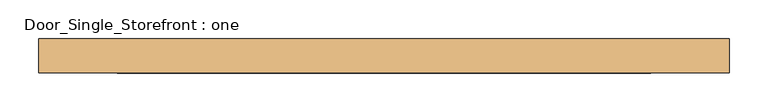
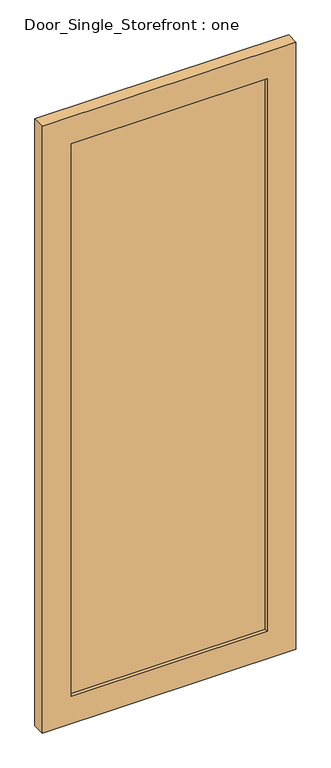
"""IFC4 building model written with IfcOpenShell, lengths in millimetres: door geometry, Door_Single_Storefront : one."""

from ifc_helpers import new_model, si_unit, frame, origin, place, context, project, spatial, polyline, outline, extrude, source, transform, mapped, element, save


def door_single_storefront_one_33456f2b(model_context):
    return source(origin(), model_context, "Body", "SweptSolid", [
        extrude(outline(polyline([(345.28125, -6.35), (-345.28125, -6.35), (-345.28125, 12.7), (345.28125, 12.7), (345.28125, -6.35)])), frame((0.0, 0.0, 101.6), z_axis=(0.0, 0.0, 1.0), x_axis=(1.0, 0.0, 0.0)), (0.0, 0.0, 1.0), 2057.4),
        extrude(outline(polyline([(2260.6, -446.88125), (0.0, -446.88125), (0.0, 446.88125), (2260.6, 446.88125), (2260.6, -446.88125)]), holes=[polyline([(101.6, 345.28125), (101.6, -345.28125), (2159.0, -345.28125), (2159.0, 345.28125), (101.6, 345.28125)])]), frame((0.0, -19.05, 0.0), z_axis=(0.0, 1.0, 0.0), x_axis=(0.0, 0.0, 1.0)), (0.0, 0.0, 1.0), 44.45),
    ])


if __name__ == "__main__":
    model = new_model("IFC4")
    model_context = context("Model", 3, world=origin())
    ifc_project = project(units=[si_unit("LENGTHUNIT", "METRE", prefix="MILLI")], contexts=[model_context])
    site = spatial("IfcSite", under=ifc_project)
    building = spatial("IfcBuilding", under=site)
    placement = place(None, origin())
    door_single_storefront_one_shape = door_single_storefront_one_33456f2b(model_context)
    element("IfcDoor", 1, ObjectType="Door_Single_Storefront : one", at=placement, inside=building, context=model_context, shape_type="MappedRepresentation", body=[
        mapped(door_single_storefront_one_shape, transform((0.0, 0.0, 0.0), x_axis=(1.0, 0.0, 0.0), y_axis=(0.0, 1.0, 0.0), z_axis=(0.0, 0.0, 1.0))),
    ])
    save(model, "model.ifc")

# Revit data of these elements
# Type "Door_Single_Storefront : one"
#   Type Mark = "27"
#   Analytic Construction = "<None>"
#   Stile_Width = 0' - 4"
#   Door_Thickness = 0' - 1 3/4"
#   Door_Offset = 0' - 1"
#   Glass_Material = Glass
#   Frame_Material = Aluminum
#   Function = (empty or 0)
# Element 1 (IfcDoor, "Door_Single_Storefront : one")
#   Materials on its faces: "Aluminum", "Glass"
# Materials
#   "Glass": class "Glass", colour RGB 142 168 196, transparency 0.75, Description = "Soda Lime Glass", Cost = 0
#   "Aluminum": class "Metal", colour RGB 226 226 226, transparency 0, Description = "Aluminum 6061", Cost = 0
